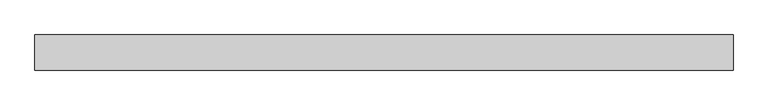
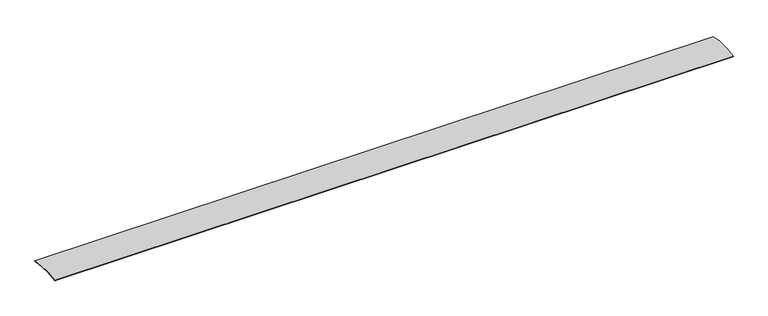
"""IFC4 building model written with IfcOpenShell, lengths in millimetres: proxy geometry, TN_ПВС 125-82_Защитная решетка : TN_ПВС 125-82_Защитная решетка."""

from ifc_helpers import new_model, si_unit, point, frame, frame_2d, origin, place, context, project, spatial, polyline, circle_curve, trimmed, segment, composite_curve, outline, extrude, source, transform, mapped, element, save


def generic_models_71aa2eb9(model_context):
    return source(origin(), model_context, "Body", "SweptSolid", [
        extrude(outline(composite_curve([segment(polyline([(-74.1, -0.0644007), (-74.1, 2.0)]), True, "CONTINUOUS"), segment(trimmed(circle_curve(frame_2d((0.0, -288.7046439)), 300.0), [point((-74.1, 2.0))], [point((74.1, 2.0))], False, "CARTESIAN"), True, "CONTINUOUS"), segment(polyline([(74.1, 2.0), (74.1, -0.0644007)]), True, "CONTINUOUS"), segment(trimmed(circle_curve(frame_2d((0.0, -288.7046439)), 298.0), [point((74.1, -0.0644007))], [point((-74.1, -0.0644007))], True, "CARTESIAN"), True, "CONTINUOUS")], self_intersect=False)), frame((0.0, 0.0, 0.0), z_axis=(1.0, 0.0, 0.0), x_axis=(0.0, 1.0, 0.0)), (0.0, 0.0, 1.0), 2942.0),
    ])


if __name__ == "__main__":
    model = new_model("IFC4")
    model_context = context("Model", 3, world=origin())
    ifc_project = project(units=[si_unit("LENGTHUNIT", "METRE", prefix="MILLI")], contexts=[model_context])
    site = spatial("IfcSite", under=ifc_project)
    building = spatial("IfcBuilding", under=site)
    placement = place(None, origin())
    generic_models_shape = generic_models_71aa2eb9(model_context)
    element("IfcBuildingElementProxy", 1, Name="TN_ПВС 125-82_Защитная решетка : TN_ПВС 125-82_Защитная решетка", ObjectType="TN_ПВС 125-82_Защитная решетка : TN_ПВС 125-82_Защитная решетка", at=placement, inside=building, context=model_context, shape_type="MappedRepresentation", body=[
        mapped(generic_models_shape, transform((0.0, 0.0, 0.0), x_axis=(1.0, 0.0, 0.0), y_axis=(0.0, 1.0, 0.0), z_axis=(0.0, 0.0, 1.0))),
    ])
    save(model, "model.ifc")

# Revit data of these elements
# Type "TN_ПВС 125-82_Защитная решетка : TN_ПВС 125-82_Защитная решетка"
#   Description = "Служит для предотвращения засора водосточной системы. Не пропускает в желоб листья и прочий крупный\r\nмусор"
#   Manufacturer = "ТехноНИКОЛЬ"
#   Model = "Комплектующие к водосточным системам"
#   URL = "https://tn-vodostok.ru/catalog/pvh/"
#   ADSK_Обозначение = "ТехноНИКОЛЬ"
#   ADSK_Наименование краткое = "Решетка"
#   ADSK_Наименование = "Защитная решетка"
#   ADSK_Масса_Текст = ""
#   ADSK_Марка = ""
#   ADSK_Код изделия = ""
#   ADSK_Завод-изготовитель = "ТехноНИКОЛЬ"
#   ADSK_Единица измерения = "п.м."
#   ADSK_Группирование = "Комплектующие к водосточным системам"
#   ADSK_URL страницы изделия = "https://tn-vodostok.ru/catalog/pvh/"
#   ADSK_URL документации изделия = "https://tn-vodostok.ru/upload/iblock/c42/c427963cb77eb5c3c51f0cfb870e9e52.pdf"
#   ADSK_Размер_Длина [instance default] = 500 mm
#   ADSK_Количество [instance default] = 0.5
#   ADSK_Материал [instance default] = TN_Пластик_Решетка_Коричневый_RAL8019
#   Default Elevation = 0
# Element 1 (IfcBuildingElementProxy, "TN_ПВС 125-82_Защитная решетка : TN_ПВС 125-82_Защитная решетка")
#   ADSK_Размер_Длина = 2942 mm
#   ADSK_Количество = 2.942
#   Materials on its faces: "TN_Пластик_Решетка_Коричневый_RAL8019"
# Materials
#   "TN_Пластик_Решетка_Коричневый_RAL8019": class "Типовые", colour RGB 61 54 53, transparency 0.25, Cost = 0
